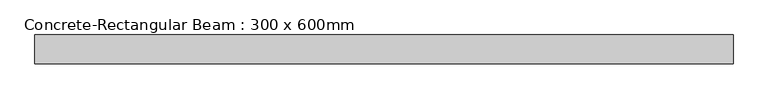
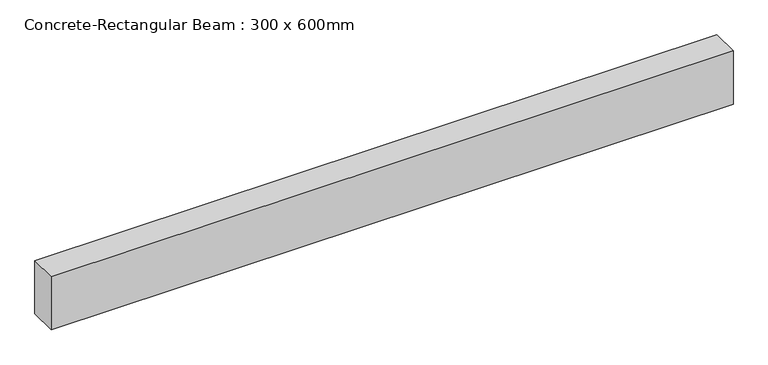
"""IFC4 building model written with IfcOpenShell, lengths in millimetres: beam geometry, Concrete-Rectangular Beam : 300 x 600mm."""

from ifc_helpers import new_model, si_unit, frame, origin, place, context, project, spatial, polyline, outline, extrude, source, transform, mapped, element, save


def concrete_rectangular_beam_300_x_600mm_2f98737b(model_context):
    return source(origin(), model_context, "Body", "SweptSolid", [
        extrude(outline(polyline([(3650.0, 150.0), (3650.0, -150.0), (-3650.0, -150.0), (-3650.0, 150.0), (3650.0, 150.0)])), frame((0.0, 0.0, -300.0), z_axis=(0.0, 0.0, 1.0), x_axis=(1.0, 0.0, 0.0)), (0.0, 0.0, 1.0), 600.0),
    ])


if __name__ == "__main__":
    model = new_model("IFC4")
    model_context = context("Model", 3, world=origin())
    ifc_project = project(units=[si_unit("LENGTHUNIT", "METRE", prefix="MILLI")], contexts=[model_context])
    site = spatial("IfcSite", under=ifc_project)
    building = spatial("IfcBuilding", under=site)
    placement = place(None, origin())
    concrete_rectangular_beam_300_x_600mm_shape = concrete_rectangular_beam_300_x_600mm_2f98737b(model_context)
    element("IfcBeam", 1, ObjectType="Concrete-Rectangular Beam : 300 x 600mm", at=placement, inside=building, context=model_context, shape_type="MappedRepresentation", body=[
        mapped(concrete_rectangular_beam_300_x_600mm_shape, transform((0.0, 0.0, 0.0), x_axis=(1.0, 0.0, 0.0), y_axis=(0.0, 1.0, 0.0), z_axis=(0.0, 0.0, 1.0))),
    ])
    save(model, "model.ifc")

# Revit data of these elements
# Type "Concrete-Rectangular Beam : 300 x 600mm"
#   Length [instance default] = 1524 mm
#   b = 300 mm
#   h = 600 mm
#   Structural Material [instance default] = Concrete, Cast-in-Place gray
#   Assembly Code = ""
# Element 1 (IfcBeam, "Concrete-Rectangular Beam : 300 x 600mm")
#   Materials on its faces: "Concrete, Cast-in-Place gray"
# Materials
#   "Concrete, Cast-in-Place gray": class "Concrete", colour RGB 192 192 192, transparency 0, Description = "Cast-in-place concrete", Cost = 0
